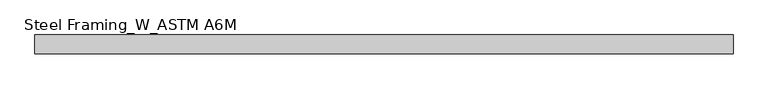
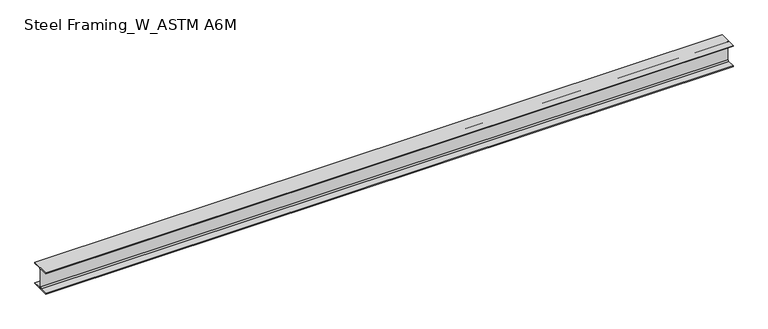
"""IFC4 building model written with IfcOpenShell, lengths in millimetres: beam geometry, Steel Framing_W_ASTM A6M : H_SB_AR_S02_W250x49.1_G5."""

from ifc_helpers import new_model, si_unit, point, frame, frame_2d, origin, place, context, project, spatial, polyline, circle_curve, trimmed, segment, composite_curve, outline, extrude, source, transform, mapped, element, save


def steel_framing_w_astm_a6m_80da07c9(model_context):
    return source(origin(), model_context, "Body", "SweptSolid", [
        extrude(outline(composite_curve([segment(polyline([(101.0, -112.5), (101.0, -123.5), (-101.0, -123.5), (-101.0, -112.5), (-16.385, -112.5)]), True, "CONTINUOUS"), segment(trimmed(circle_curve(frame_2d((-16.385, -99.8)), 12.7), [point((-16.385, -112.5))], [point((-3.685, -99.8))], True, "CARTESIAN"), True, "CONTINUOUS"), segment(polyline([(-3.685, -99.8), (-3.685, 99.8)]), True, "CONTINUOUS"), segment(trimmed(circle_curve(frame_2d((-16.385, 99.8)), 12.7), [point((-3.685, 99.8))], [point((-16.385, 112.5))], True, "CARTESIAN"), True, "CONTINUOUS"), segment(polyline([(-16.385, 112.5), (-101.0, 112.5), (-101.0, 123.5), (101.0, 123.5), (101.0, 112.5), (16.385, 112.5)]), True, "CONTINUOUS"), segment(trimmed(circle_curve(frame_2d((16.385, 99.8)), 12.7), [point((16.385, 112.5))], [point((3.685, 99.8))], True, "CARTESIAN"), True, "CONTINUOUS"), segment(polyline([(3.685, 99.8), (3.685, -99.8)]), True, "CONTINUOUS"), segment(trimmed(circle_curve(frame_2d((16.385, -99.8)), 12.7), [point((3.685, -99.8))], [point((16.385, -112.5))], True, "CARTESIAN"), True, "CONTINUOUS"), segment(polyline([(16.385, -112.5), (101.0, -112.5)]), True, "CONTINUOUS")], self_intersect=False)), frame((-3753.8, 0.0, 0.0), z_axis=(1.0, 0.0, 0.0), x_axis=(0.0, 1.0, 0.0)), (0.0, 0.0, 1.0), 7507.6),
    ])


if __name__ == "__main__":
    model = new_model("IFC4")
    model_context = context("Model", 3, world=origin())
    ifc_project = project(units=[si_unit("LENGTHUNIT", "METRE", prefix="MILLI")], contexts=[model_context])
    site = spatial("IfcSite", under=ifc_project)
    building = spatial("IfcBuilding", under=site)
    placement = place(None, origin())
    steel_framing_w_astm_a6m_shape = steel_framing_w_astm_a6m_80da07c9(model_context)
    element("IfcBeam", 1, ObjectType="Steel Framing_W_ASTM A6M : H_SB_AR_S02_W250x49.1_G5", at=placement, inside=building, context=model_context, shape_type="MappedRepresentation", body=[
        mapped(steel_framing_w_astm_a6m_shape, transform((0.0, 0.0, 0.0), x_axis=(1.0, 0.0, 0.0), y_axis=(0.0, 1.0, 0.0), z_axis=(0.0, 0.0, 1.0))),
    ])
    save(model, "model.ifc")

# Revit data of these elements
# Type "Steel Framing_W_ASTM A6M : H_SB_AR_S02_W250x49.1_G5"
#   Type Mark = "G5"
#   Section Name Key = "W10x33"
#   Width = 20.2 cm
#   Web Thickness = 0.737 cm
#   Web Fillet = 1.27 cm
#   Warping Constant = 212000.0 cm⁶
#   Torsional Moment of Inertia = 24.30 cm⁴
#   Section Area = 62.6 cm²
#   Plastic Modulus weak axis = 229.0 cm³
#   Plastic Modulus strong axis = 636.0 cm³
#   Perimeter = 1.27 m²/m
#   Nominal Weight = 49.10 kgf/m
#   Moment of Inertia weak axis = 1520.00 cm⁴
#   Moment of Inertia strong axis = 7120.00 cm⁴
#   Height = 24.7 cm
#   Flange Thickness = 1.1 cm
#   Elastic Modulus weak axis = 151.0 cm³
#   Elastic Modulus strong axis = 574.0 cm³
#   Centroid Vertical = 12.35 cm
#   Centroid Horizontal = 10.1 cm
#   Length [instance default] = 1500 mm
#   Structural Material [instance default] = Steel, 45-345
#   Bolt Spacing = 0
#   Assembly Code = ""
# Element 1 (IfcBeam, "Steel Framing_W_ASTM A6M : H_SB_AR_S02_W250x49.1_G5")
#   Materials on its faces: "Steel, 45-345"
# Materials
#   "Steel, 45-345": class "Metal", colour RGB 189 187 185, transparency 0, Description = "Steel 345 MPa", Cost = 0
